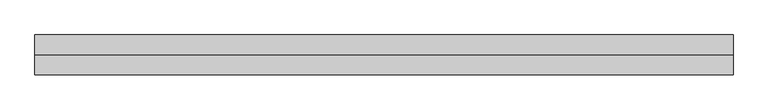
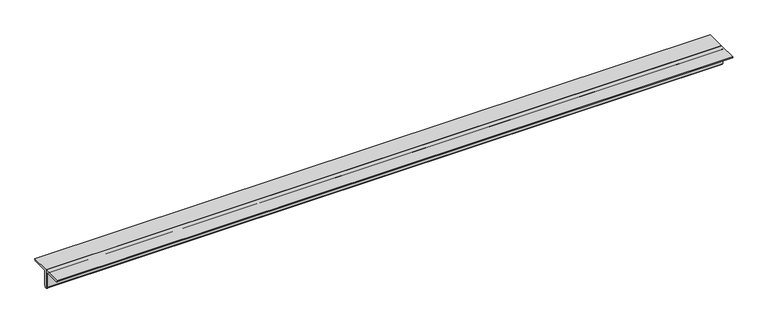
"""IFC4 building model written with IfcOpenShell, lengths in millimetres: beam geometry, 0123_Steel Framing_2Ls-KSD3502 : H_SB_AR_S04_2Ls-130x130x12_VBR1."""

from ifc_helpers import new_model, si_unit, point, frame, frame_2d, origin, place, context, project, spatial, polyline, circle_curve, trimmed, segment, composite_curve, outline, extrude, source, transform, mapped, element, save


def beam_5add8e11(model_context):
    return source(origin(), model_context, "Body", "SweptSolid", [
        extrude(outline(composite_curve([segment(polyline([(0.0, 36.4), (130.0, 36.4)]), True, "CONTINUOUS"), segment(trimmed(circle_curve(frame_2d((118.0, 36.4)), 12.0), [point((130.0, 36.4))], [point((118.0, 24.4))], False, "CARTESIAN"), True, "CONTINUOUS"), segment(polyline([(118.0, 24.4), (24.0, 24.4)]), True, "CONTINUOUS"), segment(trimmed(circle_curve(frame_2d((24.0, 12.4)), 12.0), [point((24.0, 24.4))], [point((12.0, 12.4))], True, "CARTESIAN"), True, "CONTINUOUS"), segment(polyline([(12.0, 12.4), (12.0, -81.6)]), True, "CONTINUOUS"), segment(trimmed(circle_curve(frame_2d((0.0, -81.6)), 12.0), [point((12.0, -81.6))], [point((0.0, -93.6))], False, "CARTESIAN"), True, "CONTINUOUS"), segment(polyline([(0.0, -93.6), (0.0, 36.4)]), True, "CONTINUOUS")], self_intersect=False)), frame((-2281.9000111, 0.0, 0.0), z_axis=(1.0, 0.0, 0.0), x_axis=(0.0, 1.0, 0.0)), (0.0, 0.0, 1.0), 4563.8000221),
        extrude(outline(composite_curve([segment(polyline([(0.0, 36.4), (0.0, -93.6)]), True, "CONTINUOUS"), segment(trimmed(circle_curve(frame_2d((0.0, -81.6)), 12.0), [point((0.0, -93.6))], [point((-12.0, -81.6))], False, "CARTESIAN"), True, "CONTINUOUS"), segment(polyline([(-12.0, -81.6), (-12.0, 12.4)]), True, "CONTINUOUS"), segment(trimmed(circle_curve(frame_2d((-24.0, 12.4)), 12.0), [point((-12.0, 12.4))], [point((-24.0, 24.4))], True, "CARTESIAN"), True, "CONTINUOUS"), segment(polyline([(-24.0, 24.4), (-118.0, 24.4)]), True, "CONTINUOUS"), segment(trimmed(circle_curve(frame_2d((-118.0, 36.4)), 12.0), [point((-118.0, 24.4))], [point((-130.0, 36.4))], False, "CARTESIAN"), True, "CONTINUOUS"), segment(polyline([(-130.0, 36.4), (0.0, 36.4)]), True, "CONTINUOUS")], self_intersect=False)), frame((-2281.9000111, 0.0, 0.0), z_axis=(1.0, 0.0, 0.0), x_axis=(0.0, 1.0, 0.0)), (0.0, 0.0, 1.0), 4563.8000221),
    ])


if __name__ == "__main__":
    model = new_model("IFC4")
    model_context = context("Model", 3, world=origin())
    ifc_project = project(units=[si_unit("LENGTHUNIT", "METRE", prefix="MILLI")], contexts=[model_context])
    site = spatial("IfcSite", under=ifc_project)
    building = spatial("IfcBuilding", under=site)
    placement = place(None, origin())
    beam_shape = beam_5add8e11(model_context)
    element("IfcBeam", 1, ObjectType="0123_Steel Framing_2Ls-KSD3502 : H_SB_AR_S04_2Ls-130x130x12_VBR1", at=placement, inside=building, context=model_context, shape_type="MappedRepresentation", body=[
        mapped(beam_shape, transform((0.0, 0.0, 0.0), x_axis=(1.0, 0.0, 0.0), y_axis=(0.0, 1.0, 0.0), z_axis=(0.0, 0.0, 1.0))),
    ])
    save(model, "model.ifc")

# Revit data of these elements
# Type "0123_Steel Framing_2Ls-KSD3502 : H_SB_AR_S04_2Ls-130x130x12_VBR1"
#   Type Mark = "VBR1"
#   Assembly Code = "B10"
#   Legs = "SLBB"
#   W = 8.97
#   Perimeter = 1.04 m²/m
#   Nominal Weight = 46.80 kgf/m
#   Length [instance default] = 1000 mm
#   Space = 0 mm
#   b = 130 mm
#   d = 130 mm
#   t = 12 mm
#   y = 36.4 mm
#   A = 0.005952 m²
#   Structural Material [instance default] = Steel ASTM A36
# Element 1 (IfcBeam, "0123_Steel Framing_2Ls-KSD3502 : H_SB_AR_S04_2Ls-130x130x12_VBR1")
#   Materials on its faces: "Steel ASTM A36"
# Materials
#   "Steel ASTM A36": class "Metal", colour RGB 199 199 199, transparency 0, Description = "Structural steel, ASTM A36 Grade B, mill finish", Cost = 0
